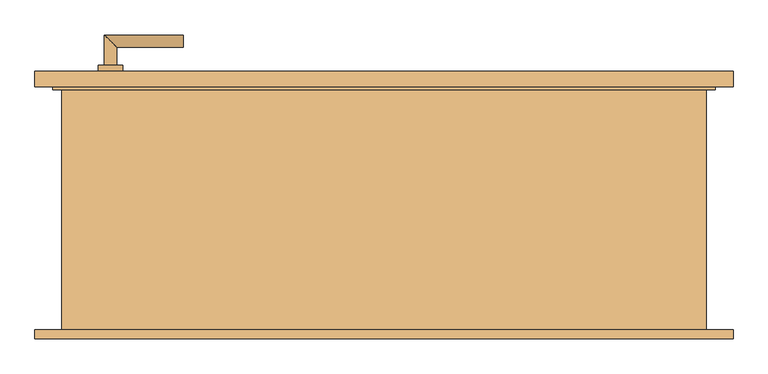
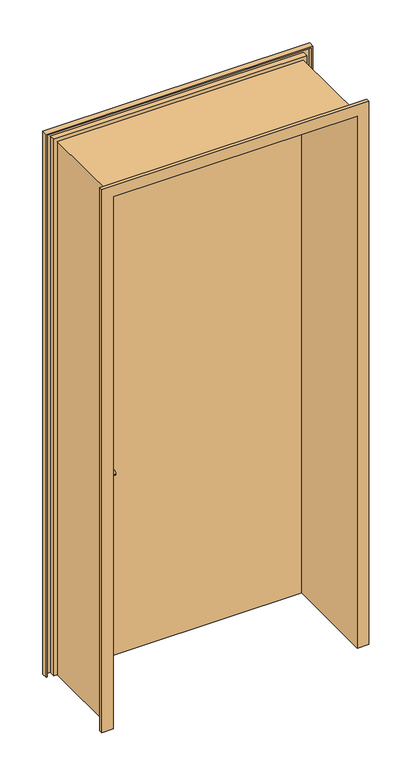
"""IFC4 building model written with IfcOpenShell, lengths in millimetres: door geometry, Drehflügel 1-flg - Stahlzarge : Glasmetalltüre 1,1 x 2,45."""

from ifc_helpers import new_model, si_unit, point, frame, frame_2d, origin, place, context, project, spatial, polyline, circle_curve, ellipse_curve, trimmed, segment, composite_curve, outline, extrude, faceted_brep, source, transform, mapped, element, save
from ifc_brep_helpers import plane_surface, cylinder_surface, advanced_brep


def door_9450e863(model_context):
    return source(origin(), model_context, "Body", "SolidModel", [
        advanced_brep(
        [(-460.0, 189.4346141, 1000.0), (-440.0, 189.4346141, 1000.0), (-460.0, 119.4346141, 1000.0), (-440.0, 139.4346141, 1000.0), (-330.0, 119.4346141, 1000.0), (-330.0, 139.4346141, 1000.0)],
        [
            (0, 1, circle_curve(frame((-450.0, 189.4346141, 1000.0), z_axis=(0.0, 1.0, 0.0), x_axis=(1.0, 0.0, 0.0)), 10.0)),
            (1, 0, circle_curve(frame((-450.0, 189.4346141, 1000.0), z_axis=(0.0, 1.0, 0.0), x_axis=(1.0, 0.0, 0.0)), 10.0)),
            (0, 2),
            (2, 3, ellipse_curve(frame((-450.0, 129.4346141, 1000.0), z_axis=(-0.7071067811865385, 0.7071067811865565, 0.0), x_axis=(0.7071067811865563, 0.7071067811865386, 0.0)), 14.1421356, 10.0)),
            (3, 1),
            (3, 2, ellipse_curve(frame((-450.0, 129.4346141, 1000.0), z_axis=(-0.7071067811865385, 0.7071067811865565, 0.0), x_axis=(0.7071067811865563, 0.7071067811865386, 0.0)), 14.1421356, 10.0)),
            (4, 5, circle_curve(frame((-330.0, 129.4346141, 1000.0), z_axis=(1.0, 0.0, 0.0), x_axis=(0.0, 1.0, 0.0)), 10.0)),
            (5, 4, circle_curve(frame((-330.0, 129.4346141, 1000.0), z_axis=(1.0, 0.0, 0.0), x_axis=(0.0, 1.0, 0.0)), 10.0)),
            (2, 4),
            (5, 3),
        ],
        [
            plane_surface(frame((-450.0, 189.4346141, -287.7526403), z_axis=(0.0, 1.0, 0.0), x_axis=(0.0, 0.0, 1.0))),
            cylinder_surface(frame((-450.0, 189.4346141, 1000.0), z_axis=(0.0, 1.0, 0.0), x_axis=(1.0, 0.0, 0.0)), 10.0),
            plane_surface(frame((-330.0, 129.4346141, -287.7526403), z_axis=(1.0, 0.0, 0.0), x_axis=(0.0, 0.0, 1.0))),
            cylinder_surface(frame((-450.0, 129.4346141, 1000.0), z_axis=(-1.0, 0.0, 0.0), x_axis=(0.0, 1.0, 0.0)), 10.0),
        ],
        [
            (0, [[1, 2]]),
            (1, [[-1, 3, 4, 5]]),
            (1, [[-2, -5, 6, -3]]),
            (2, [[7, 8]]),
            (3, [[-4, 9, -8, 10]]),
            (3, [[-6, -10, -7, -9]]),
        ],
    ),
        advanced_brep(
        [(-440.0, 249.4346141, 1000.0), (-460.0, 249.4346141, 1000.0), (-440.0, 279.4346141, 1000.0), (-460.0, 299.4346141, 1000.0), (-330.0, 279.4346141, 1000.0), (-330.0, 299.4346141, 1000.0)],
        [
            (0, 1, circle_curve(frame((-450.0, 249.4346141, 1000.0), z_axis=(0.0, -1.0, 0.0), x_axis=(-1.0, 0.0, 0.0)), 10.0)),
            (1, 0, circle_curve(frame((-450.0, 249.4346141, 1000.0), z_axis=(0.0, -1.0, 0.0), x_axis=(-1.0, 0.0, 0.0)), 10.0)),
            (0, 2),
            (2, 3, ellipse_curve(frame((-450.0, 289.4346141, 1000.0), z_axis=(-0.7071067811865475, -0.7071067811865475, 0.0), x_axis=(0.7071067811865474, -0.7071067811865476, 0.0)), 14.1421356, 10.0)),
            (3, 1),
            (3, 2, ellipse_curve(frame((-450.0, 289.4346141, 1000.0), z_axis=(-0.7071067811865475, -0.7071067811865475, 0.0), x_axis=(0.7071067811865474, -0.7071067811865476, 0.0)), 14.1421356, 10.0)),
            (4, 5, circle_curve(frame((-330.0, 289.4346141, 1000.0), z_axis=(1.0, 0.0, 0.0), x_axis=(0.0, 1.0, 0.0)), 10.0)),
            (5, 4, circle_curve(frame((-330.0, 289.4346141, 1000.0), z_axis=(1.0, 0.0, 0.0), x_axis=(0.0, 1.0, 0.0)), 10.0)),
            (2, 4),
            (5, 3),
        ],
        [
            plane_surface(frame((-450.0, 249.4346141, -287.7526403), z_axis=(0.0, -1.0, 0.0), x_axis=(0.0, 0.0, 1.0))),
            cylinder_surface(frame((-450.0, 249.4346141, 1000.0), z_axis=(0.0, -1.0, 0.0), x_axis=(-1.0, 0.0, 0.0)), 10.0),
            plane_surface(frame((-330.0, 289.4346141, -287.7526403), z_axis=(1.0, 0.0, 0.0), x_axis=(0.0, 0.0, 1.0))),
            cylinder_surface(frame((-450.0, 289.4346141, 1000.0), z_axis=(-1.0, 0.0, 0.0), x_axis=(0.0, 1.0, 0.0)), 10.0),
        ],
        [
            (0, [[1, 2]]),
            (1, [[-1, 3, 4, 5]]),
            (1, [[-2, -5, 6, -3]]),
            (2, [[7, 8]]),
            (3, [[-4, 9, -8, 10]]),
            (3, [[-6, -10, -7, -9]]),
        ],
    ),
        extrude(outline(composite_curve([segment(trimmed(circle_curve(frame_2d((1000.0, -450.0)), 20.0), [point((1000.0, -470.0))], [point((1000.0, -430.0))], False, "CARTESIAN"), True, "CONTINUOUS"), segment(trimmed(circle_curve(frame_2d((1000.0, -450.0)), 20.0), [point((1000.0, -430.0))], [point((1000.0, -470.0))], False, "CARTESIAN"), True, "CONTINUOUS")], self_intersect=False)), frame((0.0, 179.4346141, 0.0), z_axis=(0.0, 1.0, 0.0), x_axis=(0.0, 0.0, 1.0)), (0.0, 0.0, 1.0), 10.0),
        extrude(outline(composite_curve([segment(trimmed(circle_curve(frame_2d((1000.0, -450.0)), 20.0), [point((1000.0, -470.0))], [point((1000.0, -430.0))], False, "CARTESIAN"), True, "CONTINUOUS"), segment(trimmed(circle_curve(frame_2d((1000.0, -450.0)), 20.0), [point((1000.0, -430.0))], [point((1000.0, -470.0))], False, "CARTESIAN"), True, "CONTINUOUS")], self_intersect=False)), frame((0.0, 239.4346141, 0.0), z_axis=(0.0, 1.0, 0.0), x_axis=(0.0, 0.0, 1.0)), (0.0, 0.0, 1.0), 10.0),
        extrude(outline(polyline([(540.0, 214.4346141), (-540.0, 214.4346141), (-540.0, 239.4346141), (540.0, 239.4346141), (540.0, 214.4346141)])), frame((0.0, 0.0, 100.0), z_axis=(0.0, 0.0, 1.0), x_axis=(1.0, 0.0, 0.0)), (0.0, 0.0, 1.0), 2440.0),
        faceted_brep([(574.4603207, -200.5653859, 100.0), (525.0, -200.5653859, 100.0), (525.0, 214.4346141, 100.0), (540.0, 214.4346141, 100.0), (540.0, 239.4346141, 100.0), (574.4603207, 239.4346141, 100.0), (574.4603207, 214.4346141, 100.0), (569.4603207, 214.4346141, 100.0), (569.4603207, 234.4346141, 100.0), (545.0, 234.4346141, 100.0), (545.0, 209.4346141, 100.0), (530.0, 209.4346141, 100.0), (530.0, -195.5653859, 100.0), (569.4603207, -195.5653859, 100.0), (569.4603207, -185.5653859, 100.0), (574.4603207, -185.5653859, 100.0), (574.4603207, -200.5653859, 2574.4603207), (-574.4603207, -200.5653859, 2574.4603207), (-574.4603207, -200.5653859, 100.0), (-525.0, -200.5653859, 100.0), (-525.0, -200.5653859, 2525.0), (525.0, -200.5653859, 2525.0), (525.0, 214.4346141, 2525.0), (-525.0, 214.4346141, 2525.0), (-525.0, 214.4346141, 100.0), (-540.0, 214.4346141, 100.0), (-540.0, 214.4346141, 2540.0), (540.0, 214.4346141, 2540.0), (540.0, 239.4346141, 2540.0), (-540.0, 239.4346141, 2540.0), (-540.0, 239.4346141, 100.0), (-574.4603207, 239.4346141, 100.0), (-574.4603207, 239.4346141, 2574.4603207), (574.4603207, 239.4346141, 2574.4603207), (574.4603207, 214.4346141, 2574.4603207), (-574.4603207, 214.4346141, 2574.4603207), (-574.4603207, 214.4346141, 100.0), (-569.4603207, 214.4346141, 100.0), (-569.4603207, 214.4346141, 2569.4603207), (569.4603207, 214.4346141, 2569.4603207), (569.4603207, 234.4346141, 2569.4603207), (-569.4603207, 234.4346141, 2569.4603207), (-569.4603207, 234.4346141, 100.0), (-545.0, 234.4346141, 100.0), (-545.0, 234.4346141, 2545.0), (545.0, 234.4346141, 2545.0), (545.0, 209.4346141, 2545.0), (-545.0, 209.4346141, 2545.0), (-545.0, 209.4346141, 100.0), (-530.0, 209.4346141, 100.0), (-530.0, 209.4346141, 2530.0), (530.0, 209.4346141, 2530.0), (530.0, -195.5653859, 2530.0), (-530.0, -195.5653859, 2530.0), (-530.0, -195.5653859, 100.0), (-569.4603207, -195.5653859, 100.0), (-569.4603207, -195.5653859, 2569.4603207), (569.4603207, -195.5653859, 2569.4603207), (569.4603207, -185.5653859, 2569.4603207), (-569.4603207, -185.5653859, 2569.4603207), (-569.4603207, -185.5653859, 100.0), (-574.4603207, -185.5653859, 100.0), (-574.4603207, -185.5653859, 2574.4603207), (574.4603207, -185.5653859, 2574.4603207)], [[[0, 1, 2, 3, 4, 5, 6, 7, 8, 9, 10, 11, 12, 13, 14, 15]], [[1, 0, 16, 17, 18, 19, 20, 21]], [[2, 1, 21, 22]], [[3, 2, 22, 23, 24, 25, 26, 27]], [[4, 3, 27, 28]], [[5, 4, 28, 29, 30, 31, 32, 33]], [[6, 5, 33, 34]], [[7, 6, 34, 35, 36, 37, 38, 39]], [[8, 7, 39, 40]], [[9, 8, 40, 41, 42, 43, 44, 45]], [[10, 9, 45, 46]], [[11, 10, 46, 47, 48, 49, 50, 51]], [[12, 11, 51, 52]], [[13, 12, 52, 53, 54, 55, 56, 57]], [[14, 13, 57, 58]], [[15, 14, 58, 59, 60, 61, 62, 63]], [[0, 15, 63, 16]], [[17, 62, 61, 18]], [[18, 61, 60, 55, 54, 49, 48, 43, 42, 37, 36, 31, 30, 25, 24, 19]], [[23, 20, 19, 24]], [[29, 26, 25, 30]], [[35, 32, 31, 36]], [[41, 38, 37, 42]], [[47, 44, 43, 48]], [[53, 50, 49, 54]], [[59, 56, 55, 60]], [[22, 21, 20, 23]], [[28, 27, 26, 29]], [[34, 33, 32, 35]], [[40, 39, 38, 41]], [[46, 45, 44, 47]], [[52, 51, 50, 53]], [[58, 57, 56, 59]], [[16, 63, 62, 17]]]),
    ])


if __name__ == "__main__":
    model = new_model("IFC4")
    model_context = context("Model", 3, world=origin())
    ifc_project = project(units=[si_unit("LENGTHUNIT", "METRE", prefix="MILLI")], contexts=[model_context])
    site = spatial("IfcSite", under=ifc_project)
    building = spatial("IfcBuilding", under=site)
    placement = place(None, origin())
    door_shape = door_9450e863(model_context)
    element("IfcDoor", 1, ObjectType="Drehflügel 1-flg - Stahlzarge : Glasmetalltüre 1,1 x 2,45", at=placement, inside=building, context=model_context, shape_type="MappedRepresentation", body=[
        mapped(door_shape, transform((0.0, 0.0, 0.0), x_axis=(1.0, 0.0, 0.0), y_axis=(0.0, 1.0, 0.0), z_axis=(0.0, 0.0, 1.0))),
    ])
    save(model, "model.ifc")

# Revit data of these elements
# Type "Drehflügel 1-flg - Stahlzarge : Glasmetalltüre 1,1 x 2,45"
#   Type Mark = "25"
#   Operation = "SingleSwingRight"
#   Keynote = "16.03"
#   Analytic Construction = "Metall"
#   Thermal Resistance (R) = 0.270117 (m²·K)/W
#   Heat Transfer Coefficient (U) = 3.7021 W/(m²·K)
#   Rough Width = 1.100 m
#   Rough Height [instance default] = 2.550 m
#   Höhe Türgriff [instance default] = 0.900 m
#   Height = 2.450 m
#   Fußbodenaufbau [instance default] = 0.100 m
#   Width = 1.100 m
#   Sichtbarkeit Sturzlinien [instance default] = yes
#   Türgriff auswählen [instance default] = element 221079
#   Türgriff [instance default] = none
#   Türflügel [instance default] = none
#   Rahmen/Pfosten [instance default] = Metall - Lackiert - Grau
#   Visual Light Transmittance = 0
#   Solar Heat Gain Coefficient = 0
#   Function = (empty or 0)
#   Wall Closure = (empty or 0)
# Element 1 (IfcDoor, "Drehflügel 1-flg - Stahlzarge : Glasmetalltüre 1,1 x 2,45")
#   Türflügel = Holz - Bretterlage
#   Materials on its faces: "Metall - Lackiert - Grau", "Metall - Chrom", "Holz - Bretterlage"
# Materials
#   "Metall - Lackiert - Grau": class "Farbe 1", colour RGB 98 98 98, transparency 0, Cost = 0
#   "Metall - Chrom": class "Metall", colour RGB 247 247 247, transparency 0, Cost = 0
#   "Holz - Bretterlage": class "Holz", colour RGB 216 216 216, transparency 0, Cost = 0
